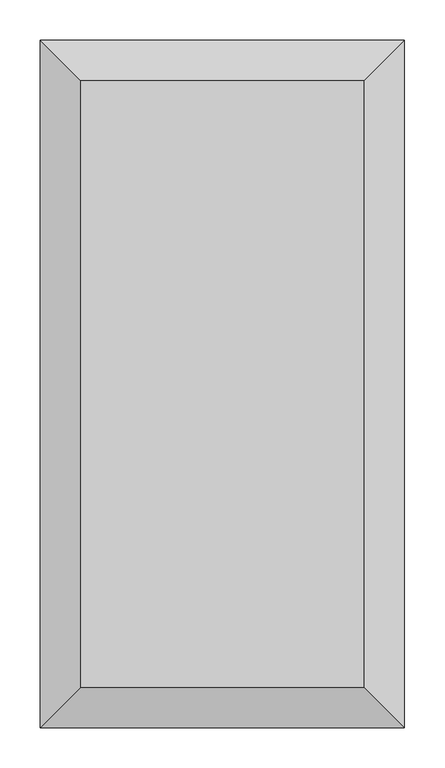
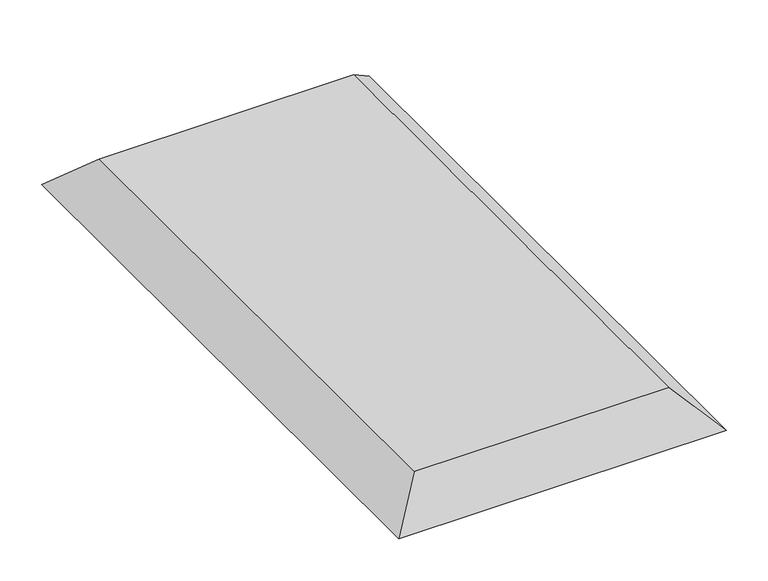
"""IFC4 building model written with IfcOpenShell, lengths in millimetres: proxy geometry, 그라우트 : 그라우트."""

from ifc_helpers import new_model, si_unit, origin, place, context, project, spatial, faceted_brep, source, transform, mapped, element, save


def generic_models_43c68623(model_context):
    return source(origin(), model_context, "Body", "Brep", [
        faceted_brep([(175.0, 375.0, 863.9720055), (-175.0, 375.0, 863.9720055), (-175.0, -375.0, 863.9720055), (175.0, -375.0, 863.9720055), (225.0, 425.0, 813.9720055), (225.0, -425.0, 813.9720055), (-225.0, -425.0, 813.9720055), (-225.0, 425.0, 813.9720055)], [[[0, 1, 2, 3]], [[4, 5, 6, 7]], [[4, 7, 1, 0]], [[7, 6, 2, 1]], [[6, 5, 3, 2]], [[5, 4, 0, 3]]]),
    ])


if __name__ == "__main__":
    model = new_model("IFC4")
    model_context = context("Model", 3, world=origin())
    ifc_project = project(units=[si_unit("LENGTHUNIT", "METRE", prefix="MILLI")], contexts=[model_context])
    site = spatial("IfcSite", under=ifc_project)
    building = spatial("IfcBuilding", under=site)
    placement = place(None, origin())
    generic_models_shape = generic_models_43c68623(model_context)
    element("IfcBuildingElementProxy", 1, Name="그라우트 : 그라우트", ObjectType="그라우트 : 그라우트", at=placement, inside=building, context=model_context, shape_type="MappedRepresentation", body=[
        mapped(generic_models_shape, transform((0.0, 0.0, 0.0), x_axis=(1.0, 0.0, 0.0), y_axis=(0.0, 1.0, 0.0), z_axis=(0.0, 0.0, 1.0))),
    ])
    save(model, "model.ifc")
